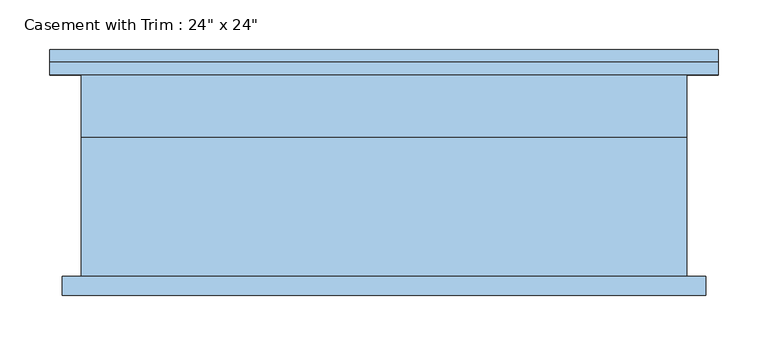
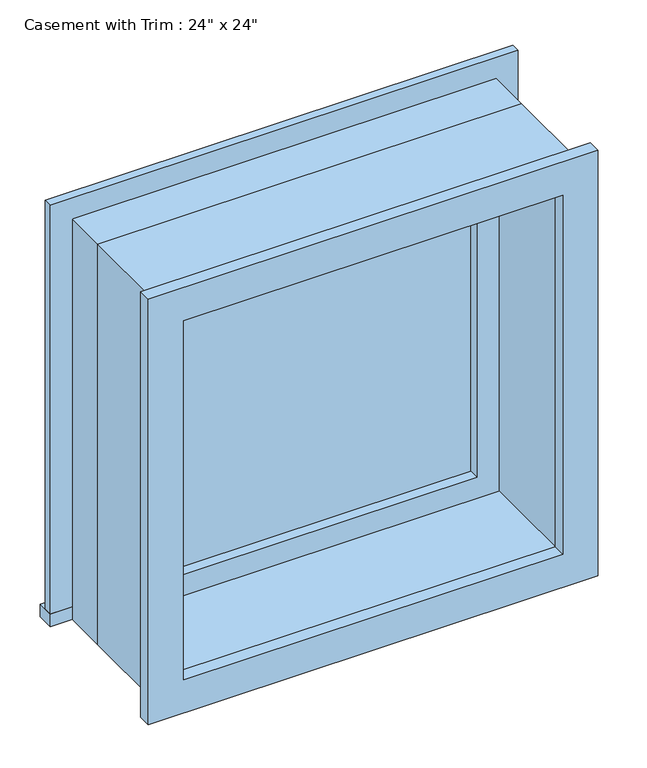
"""IFC4 building model written with IfcOpenShell, lengths in millimetres: window geometry."""

from ifc_helpers import new_model, si_unit, frame, origin, place, context, project, spatial, polyline, outline, extrude, source, transform, mapped, element, save


def window_3d989c10(model_context):
    return source(origin(), model_context, "Body", "SweptSolid", [
        extrude(outline(polyline([(-336.55, 127.0), (336.55, 127.0), (336.55, 101.6), (-336.55, 101.6), (-336.55, 127.0)])), frame((0.0, 0.0, 914.4), z_axis=(0.0, 0.0, 1.0), x_axis=(1.0, 0.0, 0.0)), (0.0, 0.0, 1.0), 19.05),
        extrude(outline(polyline([(1504.95, -285.75), (1504.95, 285.75), (933.45, 285.75), (933.45, 336.55), (1555.75, 336.55), (1555.75, -336.55), (933.45, -336.55), (933.45, -285.75), (1504.95, -285.75)])), frame((0.0, 101.6, 0.0), z_axis=(0.0, 1.0, 0.0), x_axis=(0.0, 0.0, 1.0)), (0.0, 0.0, 1.0), 12.7),
        extrude(outline(polyline([(1543.05, 323.85), (1543.05, -323.85), (895.35, -323.85), (895.35, 323.85), (1543.05, 323.85)]), holes=[polyline([(1492.25, 273.05), (946.15, 273.05), (946.15, -273.05), (1492.25, -273.05), (1492.25, 273.05)])]), frame((0.0, -120.65, 0.0), z_axis=(0.0, 1.0, 0.0), x_axis=(0.0, 0.0, 1.0)), (0.0, 0.0, 1.0), 19.05),
        extrude(outline(polyline([(241.3, 53.975), (-241.3, 53.975), (-241.3, 66.675), (241.3, 66.675), (241.3, 53.975)])), frame((0.0, 0.0, 977.9), z_axis=(0.0, 0.0, 1.0), x_axis=(1.0, 0.0, 0.0)), (0.0, 0.0, 1.0), 482.6),
        extrude(outline(polyline([(1504.95, -285.75), (933.45, -285.75), (933.45, 285.75), (1504.95, 285.75), (1504.95, -285.75)]), holes=[polyline([(1460.5, -241.3), (1460.5, 241.3), (977.9, 241.3), (977.9, -241.3), (1460.5, -241.3)])]), frame((0.0, 38.1, 0.0), z_axis=(0.0, 1.0, 0.0), x_axis=(0.0, 0.0, 1.0)), (0.0, 0.0, 1.0), 44.45),
        extrude(outline(polyline([(1524.0, -304.8), (914.4, -304.8), (914.4, 304.8), (1524.0, 304.8), (1524.0, -304.8)]), holes=[polyline([(1492.25, -273.05), (1492.25, 273.05), (946.15, 273.05), (946.15, -273.05), (1492.25, -273.05)])]), frame((0.0, -101.6, 0.0), z_axis=(0.0, 1.0, 0.0), x_axis=(0.0, 0.0, 1.0)), (0.0, 0.0, 1.0), 139.7),
        extrude(outline(polyline([(1524.0, 304.8), (1524.0, -304.8), (914.4, -304.8), (914.4, 304.8), (1524.0, 304.8)]), holes=[polyline([(1504.95, 285.75), (933.45, 285.75), (933.45, -285.75), (1504.95, -285.75), (1504.95, 285.75)])]), frame((0.0, 38.1, 0.0), z_axis=(0.0, 1.0, 0.0), x_axis=(0.0, 0.0, 1.0)), (0.0, 0.0, 1.0), 63.5),
    ])


if __name__ == "__main__":
    model = new_model("IFC4")
    model_context = context("Model", 3, world=origin())
    ifc_project = project(units=[si_unit("LENGTHUNIT", "METRE", prefix="MILLI")], contexts=[model_context])
    site = spatial("IfcSite", under=ifc_project)
    building = spatial("IfcBuilding", under=site)
    placement = place(None, origin())
    window_shape = window_3d989c10(model_context)
    element("IfcWindow", 1, ObjectType="Casement with Trim : 24\" x 24\"", at=placement, inside=building, context=model_context, shape_type="MappedRepresentation", body=[
        mapped(window_shape, transform((0.0, 0.0, 0.0), x_axis=(1.0, 0.0, 0.0), y_axis=(0.0, 1.0, 0.0), z_axis=(0.0, 0.0, 1.0))),
    ])
    save(model, "model.ifc")

# Revit data of these elements
# Type "Casement with Trim : 24\" x 24\""
#   Type Mark = "13"
#   Assembly Code = "B2020100"
#   Height = 2' - 0"
#   Default Sill Height = 3' - 0"
#   Trim Projection - Ext. = 0' - 0 1/2"
#   Trim Projection - Int. = 0' - 0 3/4"
#   Trim Width - Exterior = 0' - 2"
#   Trim Width - Interior = 0' - 2"
#   Width = 2' - 0"
#   Window Inset = 0' - 0 3/4"
#   Glass Pane Material = Glass
#   Sash Material = Sash
#   Trim Exterior Material = Trim
#   Trim Interior Material = Trim
#   Wall Closure = (empty or 0)
# Element 1 (IfcWindow, "Casement with Trim : 24\" x 24\"")
#   Materials on its faces: "Sash", "Trim", "Glass"
# Materials
#   "Glass": class "Glass", colour RGB 0 128 192, transparency 0.75
#   "Sash": class "Wood", colour RGB 224 178 126, transparency 0
#   "Trim": class "Wood", colour RGB 224 178 126, transparency 0
